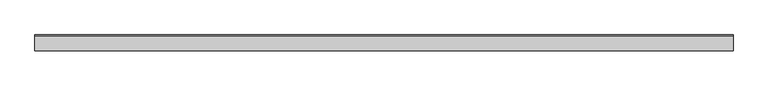
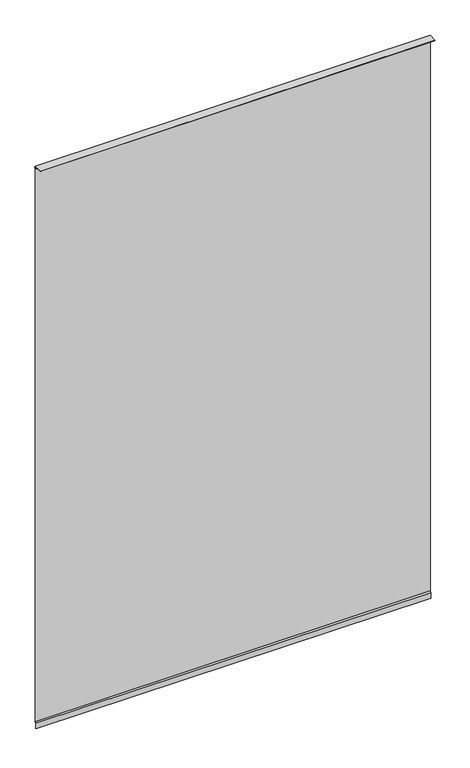
"""IFC4 building model written with IfcOpenShell, lengths in millimetres: proxy geometry, Generic Models 7:Generic Models 1:5:Generic Models 1:5 : Generic Models 7:Generic Models 1:337419:2 : Generic Models 7:Generic Models 1:5:Generic Models 1:5 : Generic Models 7:Generic Models 1:337419:311462."""

from ifc_helpers import new_model, si_unit, frame, origin, place, context, project, spatial, polyline, outline, extrude, source, transform, mapped, element, save


def generic_models_0614e2dc(model_context):
    return source(origin(), model_context, "Body", "SweptSolid", [
        extrude(outline(polyline([(-579016.439415, 3723.8950904), (-579011.2983479, 3714.990501), (-579014.9453036, 3704.9705725), (-579014.9453036, 91.1977111), (-579020.9614424, 82.6057745), (-579020.9614424, 46.3753703), (-579022.5489424, 46.3753703), (-579022.5489424, 83.1063114), (-579016.5328036, 91.698248), (-579016.5328036, 3705.2504916), (-579013.0432949, 3714.8378379), (-579017.3336513, 3722.2689531), (-579066.7458341, 3720.2101121), (-579066.8119226, 3721.7962359), (-579016.439415, 3723.8950904)])), frame((593738.0867239, 0.0, 0.0), z_axis=(1.0, 0.0, 0.0), x_axis=(0.0, 1.0, 0.0)), (0.0, 0.0, 1.0), 2444.75),
    ])


if __name__ == "__main__":
    model = new_model("IFC4")
    model_context = context("Model", 3, world=origin())
    ifc_project = project(units=[si_unit("LENGTHUNIT", "METRE", prefix="MILLI")], contexts=[model_context])
    site = spatial("IfcSite", under=ifc_project)
    building = spatial("IfcBuilding", under=site)
    placement = place(None, origin())
    generic_models_shape = generic_models_0614e2dc(model_context)
    element("IfcBuildingElementProxy", 1, Name="Generic Models 7:Generic Models 1:5:Generic Models 1:5 : Generic Models 7:Generic Models 1:337419:2 : Generic Models 7:Generic Models 1:5:Generic Models 1:5 : Generic Models 7:Generic Models 1:337419:311462", ObjectType="Generic Models 7:Generic Models 1:5:Generic Models 1:5 : Generic Models 7:Generic Models 1:337419:2 : Generic Models 7:Generic Models 1:5:Generic Models 1:5 : Generic Models 7:Generic Models 1:337419:311462", at=placement, inside=building, context=model_context, shape_type="MappedRepresentation", body=[
        mapped(generic_models_shape, transform((0.0, 0.0, 0.0), x_axis=(1.0, 0.0, 0.0), y_axis=(0.0, 1.0, 0.0), z_axis=(0.0, 0.0, 1.0))),
    ])
    save(model, "model.ifc")

# Revit data of these elements
# Type "Generic Models 7:Generic Models 1:5:Generic Models 1:5 : Generic Models 7:Generic Models 1:337419:2 : Generic Models 7:Generic Models 1:5:Generic Models 1:5 : Generic Models 7:Generic Models 1:337419:311462"
#   NameOverride = "Generic Models 7:Generic Models 1:5:Generic Models 1:5 : Generic Models 7:Generic Models 1:337419:311462"
#   ObjectTypeOverride = "Generic Models 1:5 : Generic Models 7:Generic Models 1:337419"
#   Reference = "Generic Models 1"
#   Tag = "311462"
# Element 1 (IfcBuildingElementProxy, "Generic Models 7:Generic Models 1:5:Generic Models 1:5 : Generic Models 7:Generic Models 1:337419:2 : Generic Models 7:Generic Models 1:5:Generic Models 1:5 : Generic Models 7:Generic Models 1:337419:311462")
#   Materials on its faces: "UV STABLE WATER RESISTANT VAPOR PERMEABLE AIR BARRIER"
# Materials
#   "UV STABLE WATER RESISTANT VAPOR PERMEABLE AIR BARRIER": class "Generic", colour RGB 51 162 45, transparency 0, Description = "Polyethylene film membrane", Cost = 0
